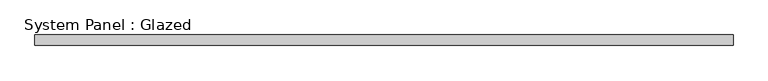
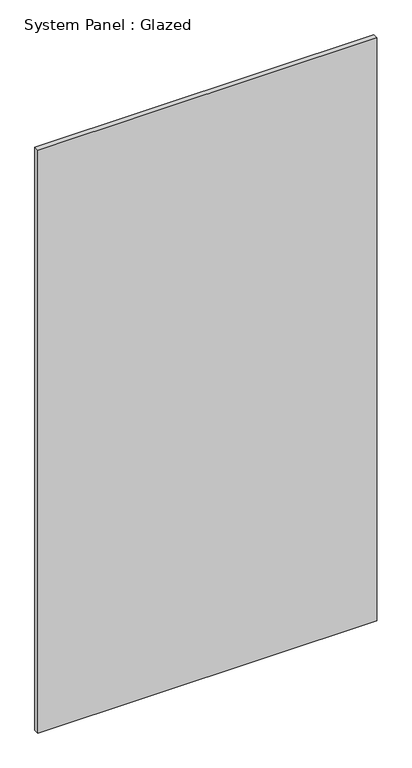
"""IFC4 building model written with IfcOpenShell, lengths in millimetres: plate geometry, System Panel : Glazed."""

from ifc_helpers import new_model, si_unit, origin, origin_with_axes, place, context, project, spatial, polyline, outline, extrude, source, transform, mapped, element, save


def system_panel_glazed_525848d0(model_context):
    return source(origin(), model_context, "Body", "SweptSolid", [
        extrude(outline(polyline([(838.1999998, 19.05), (-838.1999998, 19.05), (-838.1999998, 44.45), (838.1999998, 44.45), (838.1999998, 19.05)])), origin_with_axes(), (0.0, 0.0, 1.0), 3048.0),
    ])


if __name__ == "__main__":
    model = new_model("IFC4")
    model_context = context("Model", 3, world=origin())
    ifc_project = project(units=[si_unit("LENGTHUNIT", "METRE", prefix="MILLI")], contexts=[model_context])
    site = spatial("IfcSite", under=ifc_project)
    building = spatial("IfcBuilding", under=site)
    placement = place(None, origin())
    system_panel_glazed_shape = system_panel_glazed_525848d0(model_context)
    element("IfcPlate", 1, ObjectType="System Panel : Glazed", at=placement, inside=building, context=model_context, shape_type="MappedRepresentation", body=[
        mapped(system_panel_glazed_shape, transform((0.0, 0.0, 0.0), x_axis=(1.0, 0.0, 0.0), y_axis=(0.0, 1.0, 0.0), z_axis=(0.0, 0.0, 1.0))),
    ])
    save(model, "model.ifc")

# Revit data of these elements
# Type "System Panel : Glazed"
#   Construction Type Id = "GSP4R"
#   Analytic Construction = "1/8 in Pilkington single glazing"
#   Visual Light Transmittance = 0.9
#   Solar Heat Gain Coefficient = 0.86
#   Heat Transfer Coefficient (U) = 1.18115 BTU/(h·ft²·°F)
#   Define Thermal Properties by = 1
# Element 1 (IfcPlate, "System Panel : Glazed")
#   Materials on its faces: "Glass"
# Materials
#   "Glass": class "Glass", colour RGB 0 128 192, transparency 0.75, Description = "Soda Lime Glass", Cost = 0
